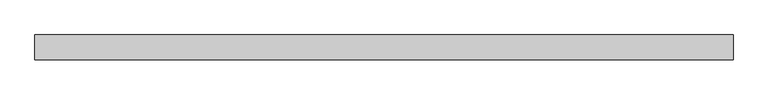
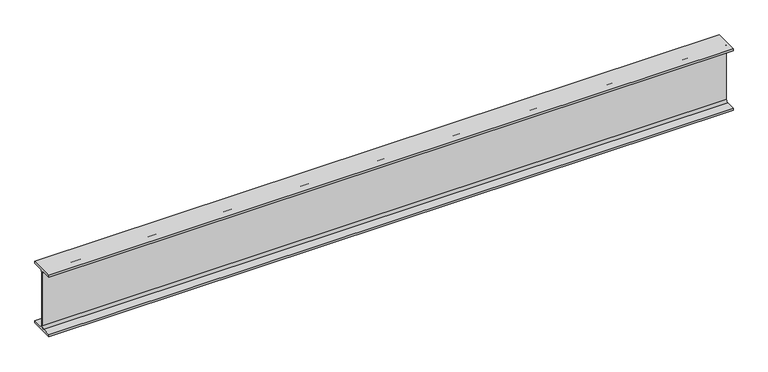
"""IFC4 building model written with IfcOpenShell, lengths in millimetres: beam geometry, 0912_Steel Framing_H-KSD3502 : H_SB_ASB_H-800x300x14x26."""

from ifc_helpers import new_model, si_unit, point, frame, frame_2d, origin, place, context, project, spatial, polyline, circle_curve, trimmed, segment, composite_curve, outline, extrude, source, transform, mapped, element, save


def beam_9f6fcf63(model_context):
    return source(origin(), model_context, "Body", "SweptSolid", [
        extrude(outline(composite_curve([segment(polyline([(150.0, -374.0), (150.0, -400.0), (-150.0, -400.0), (-150.0, -374.0), (-35.0, -374.0)]), True, "CONTINUOUS"), segment(trimmed(circle_curve(frame_2d((-35.0, -346.0)), 28.0), [point((-35.0, -374.0))], [point((-7.0, -346.0))], True, "CARTESIAN"), True, "CONTINUOUS"), segment(polyline([(-7.0, -346.0), (-7.0, 346.0)]), True, "CONTINUOUS"), segment(trimmed(circle_curve(frame_2d((-35.0, 346.0)), 28.0), [point((-7.0, 346.0))], [point((-35.0, 374.0))], True, "CARTESIAN"), True, "CONTINUOUS"), segment(polyline([(-35.0, 374.0), (-150.0, 374.0), (-150.0, 400.0), (150.0, 400.0), (150.0, 374.0), (35.0, 374.0)]), True, "CONTINUOUS"), segment(trimmed(circle_curve(frame_2d((35.0, 346.0)), 28.0), [point((35.0, 374.0))], [point((7.0, 346.0))], True, "CARTESIAN"), True, "CONTINUOUS"), segment(polyline([(7.0, 346.0), (7.0, -346.0)]), True, "CONTINUOUS"), segment(trimmed(circle_curve(frame_2d((35.0, -346.0)), 28.0), [point((7.0, -346.0))], [point((35.0, -374.0))], True, "CARTESIAN"), True, "CONTINUOUS"), segment(polyline([(35.0, -374.0), (150.0, -374.0)]), True, "CONTINUOUS")], self_intersect=False)), frame((-4157.9983828, 0.0, 0.0), z_axis=(1.0, 0.0, 0.0), x_axis=(0.0, 1.0, 0.0)), (0.0, 0.0, 1.0), 8443.8590445),
    ])


if __name__ == "__main__":
    model = new_model("IFC4")
    model_context = context("Model", 3, world=origin())
    ifc_project = project(units=[si_unit("LENGTHUNIT", "METRE", prefix="MILLI")], contexts=[model_context])
    site = spatial("IfcSite", under=ifc_project)
    building = spatial("IfcBuilding", under=site)
    placement = place(None, origin())
    beam_shape = beam_9f6fcf63(model_context)
    element("IfcBeam", 1, ObjectType="0912_Steel Framing_H-KSD3502 : H_SB_ASB_H-800x300x14x26", at=placement, inside=building, context=model_context, shape_type="MappedRepresentation", body=[
        mapped(beam_shape, transform((0.0, 0.0, 0.0), x_axis=(1.0, 0.0, 0.0), y_axis=(0.0, 1.0, 0.0), z_axis=(0.0, 0.0, 1.0))),
    ])
    save(model, "model.ifc")

# Revit data of these elements
# Type "0912_Steel Framing_H-KSD3502 : H_SB_ASB_H-800x300x14x26"
#   H_WM Code_1 = "S01AA001-00001 | Main Steel Structure Fabrication Work | Shelter/Building | Heavy Steel - Standard (Weight≥90KG/M) | Material: (   )"
#   H_WM Code_2 = "S03AA027-00001 | Main Steel Structure Erection Work | Shelter/Building | Heavy Steel (Weight≥90KG/M) | Material: (   )"
#   H_WM Code_3 = "S01AA010-00001 | Main Steel Structure Fabrication Work | Shelter/Building | Steel Painting/Coating | for Non-Fireproofed Steel Surface, Surface Preparation, Primer, Second & Final Coat | Material: (   )"
#   H_Q'ty Cal Type Tag = "SB-Q2"
#   Width = 30.0 cm
#   Web Thickness = 1.4 cm
#   Web Fillet = 2.8 cm
#   Warping Constant = 17500000.0 cm⁶
#   W = 0
#   Torsional Moment of Inertia = 422.315 cm⁴
#   Section Area = 267.4 cm²
#   Plastic Modulus weak axis = 1220.0 cm³
#   Plastic Modulus strong axis = 8240.0 cm³
#   Perimeter = 2.72 m²/m
#   Nominal Weight = 210.00 kgf/m
#   Moment of Inertia weak axis = 11700.00 cm⁴
#   Moment of Inertia strong axis = 292000.00 cm⁴
#   Height = 80.0 cm
#   Flange Thickness = 2.6 cm
#   Elastic Modulus weak axis = 782.0 cm³
#   Elastic Modulus strong axis = 7290.0 cm³
#   Centroid Vertical = 40.0 cm
#   Centroid Horizontal = 15.0 cm
#   Ix = 2920000000
#   Length [instance default] = 1.5240 m
#   Zx = 8240000
#   b = 0.3000 m
#   h = 0.8000 m
#   r = 0.0280 m
#   s = 0.0140 m
#   t = 0.0260 m
#   A = 0.02674 m²
#   Structural Material [instance default] = Steel, 45-345
#   Assembly Code = ""
# Element 1 (IfcBeam, "0912_Steel Framing_H-KSD3502 : H_SB_ASB_H-800x300x14x26")
#   Structural Material = none
# Materials
#   "Steel, 45-345": class "Metal", colour RGB 189 187 185, transparency 0, Description = "Steel 345 MPa", Cost = 0
